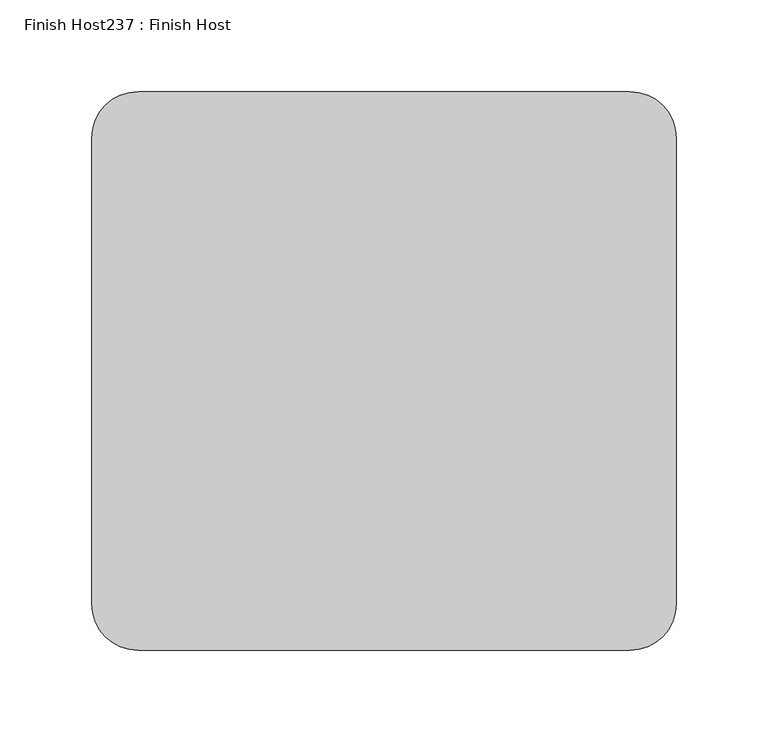
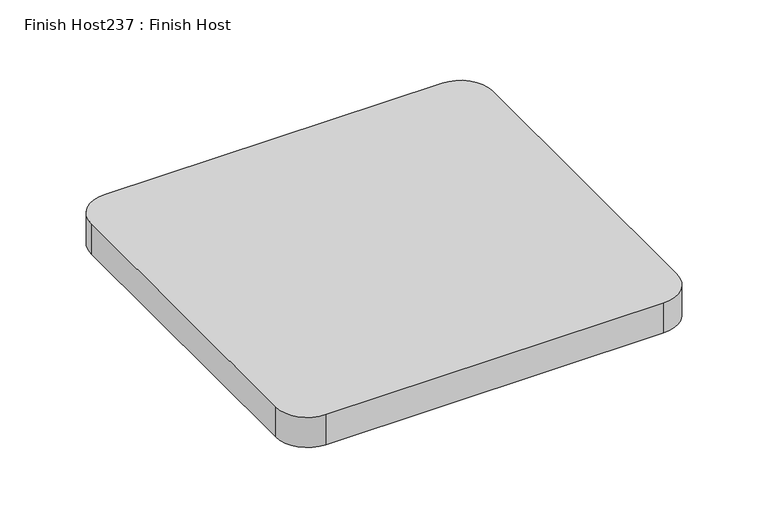
"""IFC4 building model written with IfcOpenShell, lengths in millimetres: proxy geometry, Finish Host237 : Finish Host."""

import ifcopenshell
import ifcopenshell.guid

model = None  # the IFC model being written
_history = None  # IfcOwnerHistory: only IFC2X3 demands one
_inside = {}  # id of a spatial element -> (the spatial element, [elements in it])
_under = {}  # id of a project, library or spatial element -> (it, [spatial elements below it])
_declared = {}  # id of a project -> (the project, [libraries it declares])
_typed = {}  # id of a type object -> (the type object, [elements of that type])
_made_of = {}  # id of a material, layer set ... -> (it, [elements and type objects made of it])


def new_model(schema):
    """Start an empty IFC model of exactly this schema.

    Asked for "IFC4X3", IfcOpenShell would pick the latest addendum, in which some entities
    have other attributes; the version numbers below select the first issue.
    IFC2X3 requires an IfcOwnerHistory on every rooted entity: one is made here for all.
    """
    global model, _history
    if schema == "IFC4X3":
        model = ifcopenshell.file(schema_version=(4, 3, 0, 0))
    else:
        model = ifcopenshell.file(schema=schema)
    _inside.clear()
    _under.clear()
    _declared.clear()
    _typed.clear()
    _made_of.clear()
    _history = None
    if model.schema == "IFC2X3":
        org = make("IfcOrganization", Name="unknown")
        user = make(
            "IfcPersonAndOrganization",
            ThePerson=make("IfcPerson", FamilyName="unknown"),
            TheOrganization=org,
        )
        app = make(
            "IfcApplication",
            ApplicationDeveloper=org,
            Version="unknown",
            ApplicationFullName="unknown",
            ApplicationIdentifier="unknown",
        )
        _history = make(
            "IfcOwnerHistory",
            OwningUser=user,
            OwningApplication=app,
            ChangeAction="ADDED",
            CreationDate=0,
        )
    return model


def make(cls, **values):
    """One entity of the class cls with the attributes given. An attribute that is None is left unset."""
    return model.create_entity(
        cls, **{name: value for name, value in values.items() if value is not None}
    )


def rooted(cls, **values):
    """An entity with a GlobalId (a new one), such as an element, a storey or a relation."""
    return make(cls, GlobalId=ifcopenshell.guid.new(), OwnerHistory=_history, **values)


def si_unit(unit_type, name, prefix=None):
    """IfcSIUnit, for example si_unit("LENGTHUNIT", "METRE", prefix="MILLI")."""
    return make("IfcSIUnit", UnitType=unit_type, Prefix=prefix, Name=name)


def assignment(units):
    """IfcUnitAssignment: the units of a project."""
    return None if units is None else make("IfcUnitAssignment", Units=units)


def point(xyz):
    """IfcCartesianPoint."""
    return None if xyz is None else make("IfcCartesianPoint", Coordinates=xyz)


def direction(xyz):
    """IfcDirection."""
    return None if xyz is None else make("IfcDirection", DirectionRatios=xyz)


def frame(location, z_axis=None, x_axis=None):
    """IfcAxis2Placement3D, a coordinate frame: its origin and axes. An axis left out is left unset."""
    return make(
        "IfcAxis2Placement3D",
        Location=point(location),
        Axis=direction(z_axis),
        RefDirection=direction(x_axis),
    )


def frame_2d(location, x_axis=None):
    """IfcAxis2Placement2D, a coordinate frame in the plane: its origin and x axis."""
    return make(
        "IfcAxis2Placement2D", Location=point(location), RefDirection=direction(x_axis)
    )


def origin():
    """The frame at (0, 0, 0) with its axes left unset."""
    return frame((0.0, 0.0, 0.0))


def origin_with_axes():
    """The frame at (0, 0, 0) with the z axis (0, 0, 1) and the x axis (1, 0, 0) written out."""
    return frame((0.0, 0.0, 0.0), z_axis=(0.0, 0.0, 1.0), x_axis=(1.0, 0.0, 0.0))


def place(relative_to, where):
    """IfcLocalPlacement: puts the frame where relative to a parent placement (None: the world)."""
    return make(
        "IfcLocalPlacement", PlacementRelTo=relative_to, RelativePlacement=where
    )


def context(
    kind, dimensions, precision=None, world=None, true_north=None, identifier=None
):
    """IfcGeometricRepresentationContext, for example the 3D "Model" context."""
    return make(
        "IfcGeometricRepresentationContext",
        ContextIdentifier=identifier,
        ContextType=kind,
        CoordinateSpaceDimension=dimensions,
        Precision=precision,
        WorldCoordinateSystem=world,
        TrueNorth=true_north,
    )


def project(units=None, contexts=None):
    """IfcProject with its units and contexts."""
    return rooted(
        "IfcProject",
        Name="project",
        RepresentationContexts=contexts,
        UnitsInContext=assignment(units),
    )


def spatial(cls, under=None, at=None, **own):
    """A site, building, storey or space (cls), placed at a placement, below another one or the project."""
    s = rooted(cls, ObjectPlacement=at, **own)
    if under is not None:
        _under.setdefault(under.id(), (under, []))[1].append(s)
    return s


def polyline(points):
    """IfcPolyline through the points."""
    return make("IfcPolyline", Points=[point(p) for p in points])


def circle_curve(where, radius):
    """IfcCircle in the frame where."""
    return make("IfcCircle", Position=where, Radius=radius)


def trimmed(basis, trim1, trim2, sense, master):
    """IfcTrimmedCurve: the piece of a basis curve between two trims."""
    return make(
        "IfcTrimmedCurve",
        BasisCurve=basis,
        Trim1=trim1,
        Trim2=trim2,
        SenseAgreement=sense,
        MasterRepresentation=master,
    )


def segment(curve, same_sense, transition):
    """IfcCompositeCurveSegment."""
    return make(
        "IfcCompositeCurveSegment",
        Transition=transition,
        SameSense=same_sense,
        ParentCurve=curve,
    )


def composite_curve(segments, self_intersect=None):
    """IfcCompositeCurve: segments joined end to end."""
    return make("IfcCompositeCurve", Segments=segments, SelfIntersect=self_intersect)


def outline(outer, holes=None, kind="AREA"):
    """IfcArbitraryClosedProfileDef: a profile drawn as a closed curve; with holes, ...WithVoids."""
    if holes is None:
        return make("IfcArbitraryClosedProfileDef", ProfileType=kind, OuterCurve=outer)
    return make(
        "IfcArbitraryProfileDefWithVoids",
        ProfileType=kind,
        OuterCurve=outer,
        InnerCurves=holes,
    )


def extrude(swept, where, along, depth):
    """IfcExtrudedAreaSolid: the profile swept, set in the frame where, extruded along a direction by depth."""
    return make(
        "IfcExtrudedAreaSolid",
        SweptArea=swept,
        Position=where,
        ExtrudedDirection=direction(along),
        Depth=depth,
    )


def shape(context_of_items, identifier, shape_type, items):
    """IfcShapeRepresentation: the items that make up one representation, for example the "Body"."""
    return make(
        "IfcShapeRepresentation",
        ContextOfItems=context_of_items,
        RepresentationIdentifier=identifier,
        RepresentationType=shape_type,
        Items=items,
    )


def source(mapping_origin, context_of_items, identifier, shape_type, items):
    """IfcRepresentationMap: a shape defined once, which mapped items show again and again."""
    return make(
        "IfcRepresentationMap",
        MappingOrigin=mapping_origin,
        MappedRepresentation=shape(context_of_items, identifier, shape_type, items),
    )


def transform(
    local_origin,
    x_axis=None,
    y_axis=None,
    z_axis=None,
    scale=None,
    scale2=None,
    scale3=None,
    uniform=True,
):
    """IfcCartesianTransformationOperator3D, or its non-uniform kind. x_axis, y_axis, z_axis: its Axis1, 2, 3."""
    if uniform:
        return make(
            "IfcCartesianTransformationOperator3D",
            Axis1=direction(x_axis),
            Axis2=direction(y_axis),
            LocalOrigin=point(local_origin),
            Scale=scale,
            Axis3=direction(z_axis),
        )
    return make(
        "IfcCartesianTransformationOperator3DnonUniform",
        Axis1=direction(x_axis),
        Axis2=direction(y_axis),
        LocalOrigin=point(local_origin),
        Scale=scale,
        Axis3=direction(z_axis),
        Scale2=scale2,
        Scale3=scale3,
    )


def mapped(mapping_source, mapping_target):
    """IfcMappedItem: shows the shape of a source again, moved by a transform."""
    return make(
        "IfcMappedItem", MappingSource=mapping_source, MappingTarget=mapping_target
    )


def made_of(thing, what):
    """Note that an element or type object is made of a material, layer set ...; save() writes the relation."""
    if what is not None:
        _made_of.setdefault(what.id(), (what, []))[1].append(thing)
    return thing


def element(
    cls,
    number,
    at=None,
    inside=None,
    cuts=None,
    type_object=None,
    material=None,
    context=None,
    identifier="Body",
    shape_type=None,
    held_by="IfcProductDefinitionShape",
    body=None,
    shapes=None,
    **own,
):
    """One element of the class cls, such as IfcWall. Its Tag is "e" and its number.

    at: its placement. inside: the storey or other place that contains it. cuts: it is an
    opening in that element (IfcRelVoidsElement). A single representation is given by context,
    identifier, shape_type and body (its items); several are given by shapes. held_by: the class
    of the entity that holds the representations. save() writes the other relations.
    """
    e = rooted(cls, Tag="e%d" % number, ObjectPlacement=at, **own)
    if body is not None:
        shapes = [shape(context, identifier, shape_type, body)]
    if shapes is not None:
        e.Representation = make(held_by, Representations=shapes)
    if inside is not None:
        _inside.setdefault(inside.id(), (inside, []))[1].append(e)
    if cuts is not None:
        rooted(
            "IfcRelVoidsElement", RelatingBuildingElement=cuts, RelatedOpeningElement=e
        )
    if type_object is not None:
        _typed.setdefault(type_object.id(), (type_object, []))[1].append(e)
    return made_of(e, material)


def aggregate(whole, parts):
    """IfcRelAggregates: a whole, such as a stair, and the parts it consists of."""
    return rooted("IfcRelAggregates", RelatingObject=whole, RelatedObjects=parts)


def save(model, path):
    """Write the relations noted so far, then the file.

    IfcRelAggregates (storeys below a building ...), IfcRelContainedInSpatialStructure (elements
    in a storey), IfcRelDefinesByType, IfcRelAssociatesMaterial and IfcRelDeclares: one each for
    every whole, place, type object, material and project.
    """
    for whole, parts in _under.values():
        aggregate(whole, parts)
    for where, things in _inside.values():
        rooted(
            "IfcRelContainedInSpatialStructure",
            RelatedElements=things,
            RelatingStructure=where,
        )
    for kind, things in _typed.values():
        rooted("IfcRelDefinesByType", RelatedObjects=things, RelatingType=kind)
    for what, things in _made_of.values():
        rooted("IfcRelAssociatesMaterial", RelatedObjects=things, RelatingMaterial=what)
    for by, libraries in _declared.values():
        rooted("IfcRelDeclares", RelatingContext=by, RelatedDefinitions=libraries)
    model.write(path)


def finish_host237_finish_host_53712aa4(model_context):
    return source(origin(), model_context, "Body", "SweptSolid", [
        extrude(outline(composite_curve([segment(polyline([(-49.3771625, 3462.3960864), (-49.3771625, 3716.3960864)]), True, "CONTINUOUS"), segment(trimmed(circle_curve(frame_2d((-23.9771625, 3716.3960864)), 25.4), [point((-49.3771625, 3716.3960864))], [point((-23.9771625, 3741.7960864))], False, "CARTESIAN"), True, "CONTINUOUS"), segment(polyline([(-23.9771625, 3741.7960864), (244.2157184, 3741.7960864)]), True, "CONTINUOUS"), segment(trimmed(circle_curve(frame_2d((244.2157184, 3716.3960864)), 25.4), [point((244.2157184, 3741.7960864))], [point((269.6157184, 3716.3960864))], False, "CARTESIAN"), True, "CONTINUOUS"), segment(polyline([(269.6157184, 3716.3960864), (269.6157184, 3462.3960864)]), True, "CONTINUOUS"), segment(trimmed(circle_curve(frame_2d((244.2157184, 3462.3960864)), 25.4), [point((269.6157184, 3462.3960864))], [point((244.2157184, 3436.9960864))], False, "CARTESIAN"), True, "CONTINUOUS"), segment(polyline([(244.2157184, 3436.9960864), (-23.9771625, 3436.9960864)]), True, "CONTINUOUS"), segment(trimmed(circle_curve(frame_2d((-23.9771625, 3462.3960864)), 25.4), [point((-23.9771625, 3436.9960864))], [point((-49.3771625, 3462.3960864))], False, "CARTESIAN"), True, "CONTINUOUS")], self_intersect=False)), origin_with_axes(), (0.0, 0.0, 1.0), 25.4),
    ])


if __name__ == "__main__":
    model = new_model("IFC4")
    model_context = context("Model", 3, world=origin())
    ifc_project = project(units=[si_unit("LENGTHUNIT", "METRE", prefix="MILLI")], contexts=[model_context])
    site = spatial("IfcSite", under=ifc_project)
    building = spatial("IfcBuilding", under=site)
    placement = place(None, origin())
    finish_host237_finish_host_shape = finish_host237_finish_host_53712aa4(model_context)
    element("IfcBuildingElementProxy", 1, Name="Finish Host237 : Finish Host", ObjectType="Finish Host237 : Finish Host", at=placement, inside=building, context=model_context, shape_type="MappedRepresentation", body=[
        mapped(finish_host237_finish_host_shape, transform((0.0, 0.0, 0.0), x_axis=(1.0, 0.0, 0.0), y_axis=(0.0, 1.0, 0.0), z_axis=(0.0, 0.0, 1.0))),
    ])
    save(model, "model.ifc")

# Revit data of these elements
# Type "Finish Host237 : Finish Host"
#   Countertop Material = Fabric - Teknion - P406 - Peru - Cuzco
# Element 1 (IfcBuildingElementProxy, "Finish Host237 : Finish Host")
#   Materials on its faces: "Fabric - Teknion - P406 - Peru - Cuzco"
# Materials
#   "Fabric - Teknion - P406 - Peru - Cuzco": class "Fabric", colour RGB 45 45 45, transparency 0, Model = "P406", Manufacturer = "Teknion Studio", URL = "http://www.teknionstudio.com/", Description = "Cuzco Peru", Cost = 0
